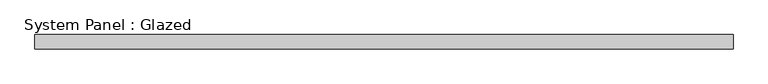
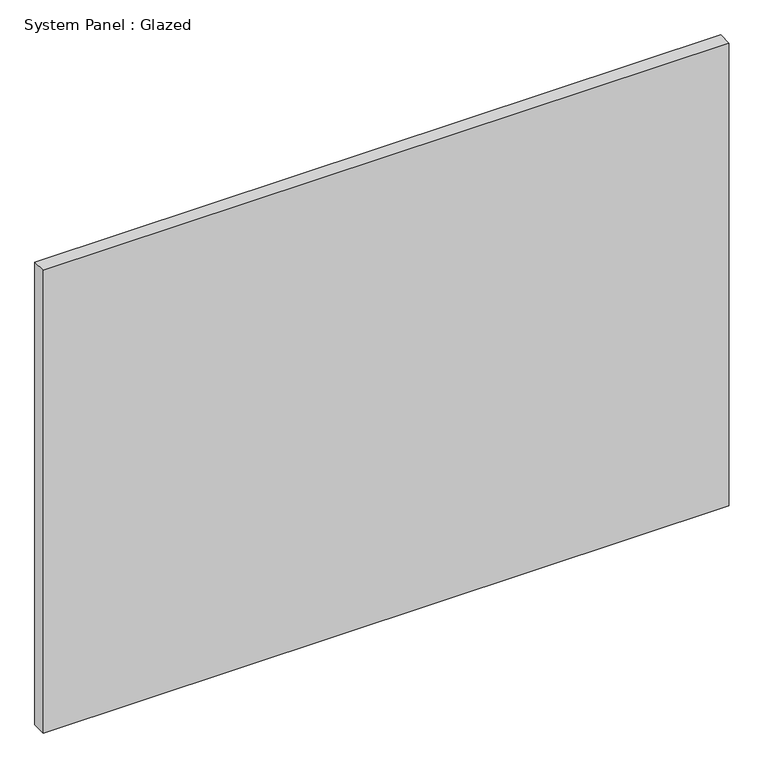
"""IFC4 building model written with IfcOpenShell, lengths in millimetres: plate geometry, System Panel : Glazed."""

from ifc_helpers import new_model, si_unit, origin, origin_with_axes, place, context, project, spatial, polyline, outline, extrude, source, transform, mapped, element, save


def system_panel_glazed_f4c55b59(model_context):
    return source(origin(), model_context, "Body", "SweptSolid", [
        extrude(outline(polyline([(610.2825643, 19.05), (-610.2825643, 19.05), (-610.2825643, 44.45), (610.2825643, 44.45), (610.2825643, 19.05)])), origin_with_axes(), (0.0, 0.0, 1.0), 869.95),
    ])


if __name__ == "__main__":
    model = new_model("IFC4")
    model_context = context("Model", 3, world=origin())
    ifc_project = project(units=[si_unit("LENGTHUNIT", "METRE", prefix="MILLI")], contexts=[model_context])
    site = spatial("IfcSite", under=ifc_project)
    building = spatial("IfcBuilding", under=site)
    placement = place(None, origin())
    system_panel_glazed_shape = system_panel_glazed_f4c55b59(model_context)
    element("IfcPlate", 1, ObjectType="System Panel : Glazed", at=placement, inside=building, context=model_context, shape_type="MappedRepresentation", body=[
        mapped(system_panel_glazed_shape, transform((0.0, 0.0, 0.0), x_axis=(1.0, 0.0, 0.0), y_axis=(0.0, 1.0, 0.0), z_axis=(0.0, 0.0, 1.0))),
    ])
    save(model, "model.ifc")

# Revit data of these elements
# Element 1 (IfcPlate, "System Panel : Glazed")
#   Materials on its faces: "Glass"
# Materials
#   "Glass": class "Glass", colour RGB 0 128 192, transparency 0.75
